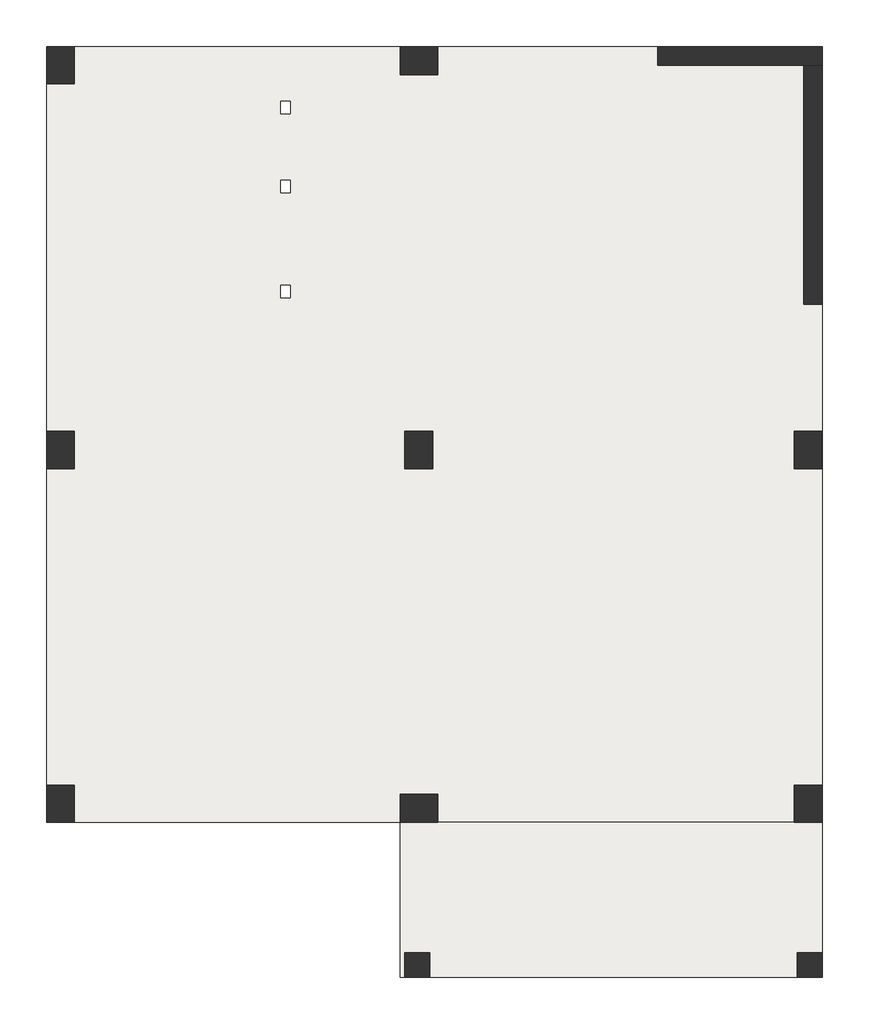
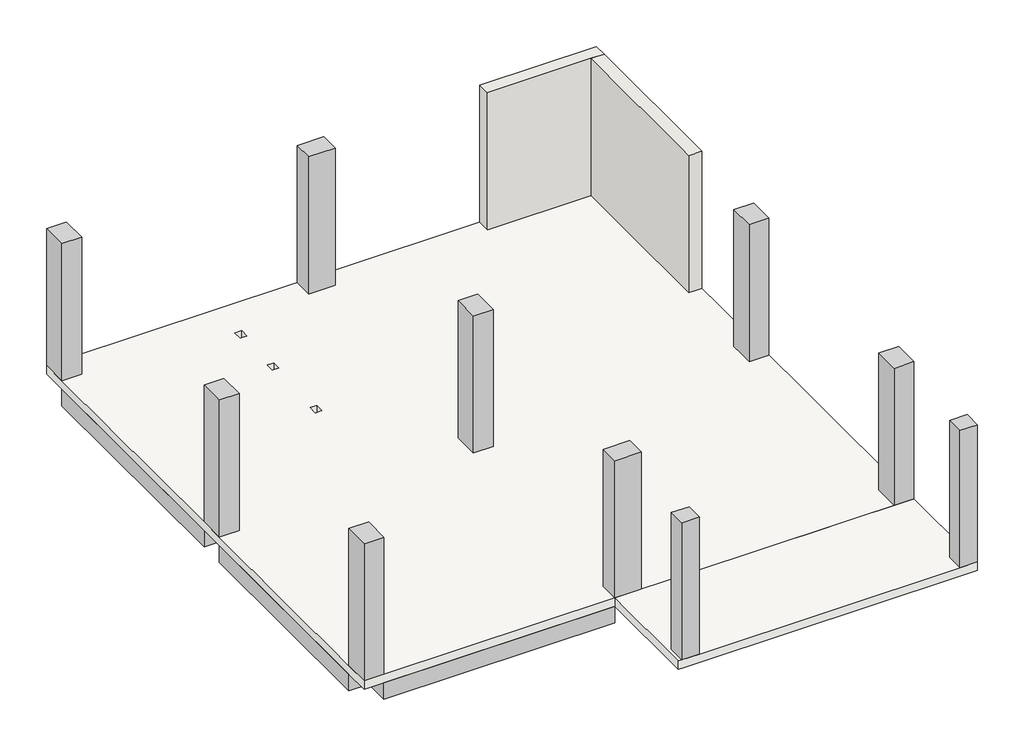
# One storey: 12 beams, 10 columns, 2 slabs, 2 walls.
"""IFC4 building model written with IfcOpenShell, lengths in millimetres."""

from ifc_helpers import new_model, si_unit, frame, origin, place, context, project, spatial, polyline, outline, extrude, faceted_brep, element, save

model = new_model("IFC4")

# Units and contexts
model_context = context("Model", 3, world=origin())
ifc_project = project(units=[si_unit("LENGTHUNIT", "METRE", prefix="MILLI")], contexts=[model_context])

# Site, building, storey
site = spatial("IfcSite", under=ifc_project)
building = spatial("IfcBuilding", under=site)
storey = spatial("IfcBuildingStorey", under=building, Name="01 Birinci Kat", Elevation=97280.0)

# Beams
placement = place(None, origin())
element("IfcBeam", 1, ObjectType="M_Concrete-Rectangular Beam : 45x60cm Kiriş", at=placement, inside=storey, context=model_context, shape_type="SweptSolid", body=[
    extrude(outline(polyline([(6225.0, 14999.2150597), (5700.0, 14999.2150597), (5700.0, 14550.0), (450.0, 14550.0), (450.0, 15000.0), (6225.0, 15000.0), (6225.0, 14999.2150597)])), frame((0.0, 0.0, 96680.0), z_axis=(0.0, 0.0, 1.0), x_axis=(1.0, 0.0, 0.0)), (0.0, 0.0, 1.0), 400.0),
])
element("IfcBeam", 2, ObjectType="M_Concrete-Rectangular Beam : 45x60cm Kiriş", at=placement, inside=storey, context=model_context, shape_type="SweptSolid", body=[
    extrude(outline(polyline([(450.0, 8750.0), (5775.0, 8750.0), (5775.0, 8300.0), (450.0, 8300.0), (450.0, 8750.0)])), frame((0.0, 0.0, 96680.0), z_axis=(0.0, 0.0, 1.0), x_axis=(1.0, 0.0, 0.0)), (0.0, 0.0, 1.0), 400.0),
])
element("IfcBeam", 3, ObjectType="M_Concrete-Rectangular Beam : 45x60cm Kiriş", at=placement, inside=storey, context=model_context, shape_type="SweptSolid", body=[
    extrude(outline(polyline([(0.0, 8800.0), (0.0, 14400.0), (450.0, 14400.0), (450.0, 8800.0), (0.0, 8800.0)])), frame((0.0, 0.0, 96680.0), z_axis=(0.0, 0.0, 1.0), x_axis=(1.0, 0.0, 0.0)), (0.0, 0.0, 1.0), 400.0),
])
element("IfcBeam", 4, ObjectType="M_Concrete-Rectangular Beam : 45x60cm Kiriş", at=placement, inside=storey, context=model_context, shape_type="SweptSolid", body=[
    extrude(outline(polyline([(0.0, 3100.0), (0.0, 8200.0), (450.0, 8200.0), (450.0, 3100.0), (0.0, 3100.0)])), frame((0.0, 0.0, 96680.0), z_axis=(0.0, 0.0, 1.0), x_axis=(1.0, 0.0, 0.0)), (0.0, 0.0, 1.0), 400.0),
])
element("IfcBeam", 5, ObjectType="M_Concrete-Rectangular Beam : 45x60cm Kiriş", at=placement, inside=storey, context=model_context, shape_type="SweptSolid", body=[
    extrude(outline(polyline([(5700.0, 2500.0), (450.0, 2500.0), (450.0, 2950.0), (5700.0, 2950.0), (5700.0, 2500.0)])), frame((0.0, 0.0, 96680.0), z_axis=(0.0, 0.0, 1.0), x_axis=(1.0, 0.0, 0.0)), (0.0, 0.0, 1.0), 400.0),
])
element("IfcBeam", 6, ObjectType="M_Concrete-Rectangular Beam : 45x60cm Kiriş", at=placement, inside=storey, context=model_context, shape_type="SweptSolid", body=[
    extrude(outline(polyline([(12050.0, 2500.0), (6300.0, 2500.0), (6300.0, 2950.0), (12050.0, 2950.0), (12050.0, 2500.0)])), frame((0.0, 0.0, 96680.0), z_axis=(0.0, 0.0, 1.0), x_axis=(1.0, 0.0, 0.0)), (0.0, 0.0, 1.0), 400.0),
])
element("IfcBeam", 7, ObjectType="M_Concrete-Rectangular Beam : 45x60cm Kiriş", at=placement, inside=storey, context=model_context, shape_type="SweptSolid", body=[
    extrude(outline(polyline([(12500.0, 8750.0), (12500.0, 3100.0), (12050.0, 3100.0), (12050.0, 8200.0), (12494.8117928, 8200.0), (12494.8117928, 8750.0), (12500.0, 8750.0)])), frame((0.0, 0.0, 96680.0), z_axis=(0.0, 0.0, 1.0), x_axis=(1.0, 0.0, 0.0)), (0.0, 0.0, 1.0), 400.0),
])
element("IfcBeam", 8, ObjectType="M_Concrete-Rectangular Beam : 45x60cm Kiriş", at=placement, inside=storey, context=model_context, shape_type="SweptSolid", body=[
    extrude(outline(polyline([(12044.8117928, 8750.0), (12044.8117928, 8300.0), (6237.7, 8300.0), (6237.7, 8750.0), (12044.8117928, 8750.0)])), frame((0.0, 0.0, 96680.0), z_axis=(0.0, 0.0, 1.0), x_axis=(1.0, 0.0, 0.0)), (0.0, 0.0, 1.0), 400.0),
])
element("IfcBeam", 9, ObjectType="M_Concrete-Rectangular Beam : 30x60cm Kiriş", at=placement, inside=storey, context=model_context, shape_type="SweptSolid", body=[
    extrude(outline(polyline([(9850.0, 15000.0), (9850.0, 14700.0), (6300.0, 14700.0), (6300.0, 15000.0), (9850.0, 15000.0)])), frame((0.0, 0.0, 96680.0), z_axis=(0.0, 0.0, 1.0), x_axis=(1.0, 0.0, 0.0)), (0.0, 0.0, 1.0), 400.0),
])
element("IfcBeam", 10, ObjectType="M_Concrete-Rectangular Beam : 30x60cm Kiriş", at=placement, inside=storey, context=model_context, shape_type="SweptSolid", body=[
    extrude(outline(polyline([(12200.0, 10850.0), (12500.0, 10850.0), (12500.0, 8800.0), (12200.0, 8800.0), (12200.0, 10850.0)])), frame((0.0, 0.0, 96680.0), z_axis=(0.0, 0.0, 1.0), x_axis=(1.0, 0.0, 0.0)), (0.0, 0.0, 1.0), 400.0),
])
element("IfcBeam", 11, ObjectType="M_Concrete-Rectangular Beam : 45x60cm Kiriş", at=placement, inside=storey, context=model_context, shape_type="SweptSolid", body=[
    extrude(outline(polyline([(5775.0, 2950.0), (5775.0, 8200.0), (6225.0, 8200.0), (6225.0, 2950.0), (5775.0, 2950.0)])), frame((0.0, 0.0, 96680.0), z_axis=(0.0, 0.0, 1.0), x_axis=(1.0, 0.0, 0.0)), (0.0, 0.0, 1.0), 400.0),
])
element("IfcBeam", 12, ObjectType="M_Concrete-Rectangular Beam : 45x60cm Kiriş", at=placement, inside=storey, context=model_context, shape_type="SweptSolid", body=[
    extrude(outline(polyline([(5775.0, 14536.5150597), (6225.0, 14536.5150597), (6225.0, 8800.0), (5775.0, 8800.0), (5775.0, 14536.5150597)])), frame((0.0, 0.0, 96680.0), z_axis=(0.0, 0.0, 1.0), x_axis=(1.0, 0.0, 0.0)), (0.0, 0.0, 1.0), 400.0),
])

# Columns
element("IfcColumn", 13, ObjectType="M_Concrete-Rectangular-Column : 45x60cm Kolon", at=placement, inside=storey, context=model_context, shape_type="SweptSolid", body=[
    extrude(outline(polyline([(0.0, 14400.0), (0.0, 15000.0), (450.0, 15000.0), (450.0, 14400.0), (0.0, 14400.0)])), frame((0.0, 0.0, 97280.0), z_axis=(0.0, 0.0, 1.0), x_axis=(1.0, 0.0, 0.0)), (0.0, 0.0, 1.0), 3300.0),
])
element("IfcColumn", 14, ObjectType="M_Concrete-Rectangular-Column : 45x60cm Kolon", at=placement, inside=storey, context=model_context, shape_type="SweptSolid", body=[
    extrude(outline(polyline([(5700.0, 14999.2150597), (6300.0, 14999.2150597), (6300.0, 14549.2150597), (5700.0, 14549.2150597), (5700.0, 14999.2150597)])), frame((0.0, 0.0, 97280.0), z_axis=(0.0, 0.0, 1.0), x_axis=(1.0, 0.0, 0.0)), (0.0, 0.0, 1.0), 3300.0),
])
element("IfcColumn", 15, ObjectType="M_Concrete-Rectangular-Column : 45x60cm Kolon", at=placement, inside=storey, context=model_context, shape_type="SweptSolid", body=[
    extrude(outline(polyline([(450.0, 8800.0), (450.0, 8200.0), (0.0, 8200.0), (0.0, 8800.0), (450.0, 8800.0)])), frame((0.0, 0.0, 97280.0), z_axis=(0.0, 0.0, 1.0), x_axis=(1.0, 0.0, 0.0)), (0.0, 0.0, 1.0), 3300.0),
])
element("IfcColumn", 16, ObjectType="M_Concrete-Rectangular-Column : 45x60cm Kolon", at=placement, inside=storey, context=model_context, shape_type="SweptSolid", body=[
    extrude(outline(polyline([(6225.0, 8800.0), (6225.0, 8200.0), (5775.0, 8200.0), (5775.0, 8800.0), (6225.0, 8800.0)])), frame((0.0, 0.0, 97280.0), z_axis=(0.0, 0.0, 1.0), x_axis=(1.0, 0.0, 0.0)), (0.0, 0.0, 1.0), 3300.0),
])
element("IfcColumn", 17, ObjectType="M_Concrete-Rectangular-Column : 45x60cm Kolon", at=placement, inside=storey, context=model_context, shape_type="SweptSolid", body=[
    extrude(outline(polyline([(12494.8117928, 8800.0), (12494.8117928, 8200.0), (12044.8117928, 8200.0), (12044.8117928, 8800.0), (12494.8117928, 8800.0)])), frame((0.0, 0.0, 97280.0), z_axis=(0.0, 0.0, 1.0), x_axis=(1.0, 0.0, 0.0)), (0.0, 0.0, 1.0), 3300.0),
])
element("IfcColumn", 18, ObjectType="M_Concrete-Rectangular-Column : 45x60cm Kolon", at=placement, inside=storey, context=model_context, shape_type="SweptSolid", body=[
    extrude(outline(polyline([(12500.0, 3100.0), (12500.0, 2500.0), (12050.0, 2500.0), (12050.0, 3100.0), (12500.0, 3100.0)])), frame((0.0, 0.0, 97280.0), z_axis=(0.0, 0.0, 1.0), x_axis=(1.0, 0.0, 0.0)), (0.0, 0.0, 1.0), 3300.0),
])
element("IfcColumn", 19, ObjectType="M_Concrete-Rectangular-Column : 45x60cm Kolon", at=placement, inside=storey, context=model_context, shape_type="SweptSolid", body=[
    extrude(outline(polyline([(450.0, 3100.0), (450.0, 2500.0), (0.0, 2500.0), (0.0, 3100.0), (450.0, 3100.0)])), frame((0.0, 0.0, 97280.0), z_axis=(0.0, 0.0, 1.0), x_axis=(1.0, 0.0, 0.0)), (0.0, 0.0, 1.0), 3300.0),
])
element("IfcColumn", 20, ObjectType="M_Concrete-Rectangular-Column : 45x60cm Kolon", at=placement, inside=storey, context=model_context, shape_type="SweptSolid", body=[
    extrude(outline(polyline([(5700.0, 2950.0), (6300.0, 2950.0), (6300.0, 2500.0), (5700.0, 2500.0), (5700.0, 2950.0)])), frame((0.0, 0.0, 97280.0), z_axis=(0.0, 0.0, 1.0), x_axis=(1.0, 0.0, 0.0)), (0.0, 0.0, 1.0), 3300.0),
])
element("IfcColumn", 21, ObjectType="M_Concrete-Rectangular-Column : 40x40cm Kolon", at=placement, inside=storey, context=model_context, shape_type="SweptSolid", body=[
    extrude(outline(polyline([(6175.0, 400.0), (6175.0, 0.0), (5775.0, 0.0), (5775.0, 400.0), (6175.0, 400.0)])), frame((0.0, 0.0, 97280.0), z_axis=(0.0, 0.0, 1.0), x_axis=(1.0, 0.0, 0.0)), (0.0, 0.0, 1.0), 3300.0),
])
element("IfcColumn", 22, ObjectType="M_Concrete-Rectangular-Column : 40x40cm Kolon", at=placement, inside=storey, context=model_context, shape_type="SweptSolid", body=[
    extrude(outline(polyline([(12500.0, 400.0), (12500.0, 0.0), (12100.0, 0.0), (12100.0, 400.0), (12500.0, 400.0)])), frame((0.0, 0.0, 97280.0), z_axis=(0.0, 0.0, 1.0), x_axis=(1.0, 0.0, 0.0)), (0.0, 0.0, 1.0), 3300.0),
])

# Slabs
element("IfcSlab", 23, ObjectType="20cm Döşeme", at=placement, inside=storey, context=model_context, shape_type="Brep", body=[
    faceted_brep([(12500.0, 15000.0, 97080.0), (12500.0, 10850.0, 97080.0), (12500.0, 8800.0, 97080.0), (12500.0, 8750.0, 97080.0), (12500.0, 3100.0, 97080.0), (12500.0, 2500.0, 97080.0), (12050.0, 2500.0, 97080.0), (6300.0, 2500.0, 97080.0), (5700.0, 2500.0, 97080.0), (450.0, 2500.0, 97080.0), (0.0, 2500.0, 97080.0), (0.0, 3100.0, 97080.0), (0.0, 8200.0, 97080.0), (0.0, 8800.0, 97080.0), (0.0, 14400.0, 97080.0), (0.0, 15000.0, 97080.0), (450.0, 15000.0, 97080.0), (6225.0, 15000.0, 97080.0), (6300.0, 15000.0, 97080.0), (9850.0, 15000.0, 97080.0), (3925.0, 14120.0, 97080.0), (3775.0, 14120.0, 97080.0), (3775.0, 13920.0, 97080.0), (3925.0, 13920.0, 97080.0), (3925.0, 12846.5789726, 97080.0), (3775.0, 12846.5789726, 97080.0), (3775.0, 12646.5789726, 97080.0), (3925.0, 12646.5789726, 97080.0), (3775.0, 10954.975, 97080.0), (3925.0, 10954.975, 97080.0), (3925.0, 11154.975, 97080.0), (3775.0, 11154.975, 97080.0), (12500.0, 15000.0, 97280.0), (450.0, 15000.0, 97280.0), (0.0, 15000.0, 97280.0), (0.0, 14400.0, 97280.0), (0.0, 8800.0, 97280.0), (0.0, 8200.0, 97280.0), (0.0, 3100.0, 97280.0), (0.0, 2500.0, 97280.0), (450.0, 2500.0, 97280.0), (5700.0, 2500.0, 97280.0), (6300.0, 2500.0, 97280.0), (12050.0, 2500.0, 97280.0), (12500.0, 2500.0, 97280.0), (12500.0, 3100.0, 97280.0), (3925.0, 14120.0, 97280.0), (3925.0, 13920.0, 97280.0), (3775.0, 13920.0, 97280.0), (3775.0, 14120.0, 97280.0), (3925.0, 12846.5789726, 97280.0), (3925.0, 12646.5789726, 97280.0), (3775.0, 12646.5789726, 97280.0), (3775.0, 12846.5789726, 97280.0), (3775.0, 10954.975, 97280.0), (3775.0, 11154.975, 97280.0), (3925.0, 11154.975, 97280.0), (3925.0, 10954.975, 97280.0)], [[[0, 1, 2, 3, 4, 5, 6, 7, 8, 9, 10, 11, 12, 13, 14, 15, 16, 17, 18, 19], [20, 21, 22, 23], [24, 25, 26, 27], [28, 29, 30, 31]], [[32, 33, 34, 35, 36, 37, 38, 39, 40, 41, 42, 43, 44, 45], [46, 47, 48, 49], [50, 51, 52, 53], [54, 55, 56, 57]], [[5, 4, 3, 2, 1, 0, 32, 45, 44]], [[10, 9, 8, 7, 6, 5, 44, 43, 42, 41, 40, 39]], [[15, 14, 13, 12, 11, 10, 39, 38, 37, 36, 35, 34]], [[0, 19, 18, 17, 16, 15, 34, 33, 32]], [[21, 20, 46, 49]], [[22, 21, 49, 48]], [[23, 22, 48, 47]], [[20, 23, 47, 46]], [[25, 24, 50, 53]], [[26, 25, 53, 52]], [[27, 26, 52, 51]], [[24, 27, 51, 50]], [[29, 28, 54, 57]], [[30, 29, 57, 56]], [[31, 30, 56, 55]], [[28, 31, 55, 54]]]),
])
element("IfcSlab", 24, ObjectType="20cm Döşeme", at=placement, inside=storey, context=model_context, shape_type="Brep", body=[
    faceted_brep([(12500.0, 2500.0, 97080.0), (12500.0, 450.0, 97080.0), (12500.0, 0.0, 97080.0), (12050.0, 0.0, 97080.0), (6225.0, 0.0, 97080.0), (5775.0, 0.0, 97080.0), (5700.0, 0.0, 97080.0), (5700.0, 2500.0, 97080.0), (12500.0, 2500.0, 97280.0), (5700.0, 2500.0, 97280.0), (5700.0, 0.0, 97280.0), (5775.0, 0.0, 97280.0), (6175.0, 0.0, 97280.0), (12100.0, 0.0, 97280.0), (12500.0, 0.0, 97280.0), (12500.0, 400.0, 97280.0)], [[[0, 1, 2, 3, 4, 5, 6, 7]], [[8, 9, 10, 11, 12, 13, 14, 15]], [[2, 1, 0, 8, 15, 14]], [[6, 5, 4, 3, 2, 14, 13, 12, 11, 10]], [[7, 6, 10, 9]], [[0, 7, 9, 8]]]),
])

# Walls
element("IfcWall", 25, ObjectType="30cm Perde Duvar", at=placement, inside=storey, context=model_context, shape_type="Brep", body=[
    faceted_brep([(9850.0, 14700.0, 97280.0), (12200.0, 14700.0, 97280.0), (12500.0, 14700.0, 97280.0), (12500.0, 14700.0, 100580.0), (12200.0, 14700.0, 100580.0), (9850.0, 14700.0, 100580.0), (9850.0, 14700.0, 100180.0), (9850.0, 15000.0, 97280.0), (9850.0, 15000.0, 100180.0), (9850.0, 15000.0, 100580.0), (12500.0, 15000.0, 100580.0), (12500.0, 15000.0, 97280.0)], [[[0, 1, 2, 3, 4, 5, 6]], [[7, 8, 9, 10, 11]], [[2, 1, 0, 7, 11]], [[0, 6, 5, 9, 8, 7]], [[3, 2, 11, 10]], [[5, 4, 3, 10, 9]]]),
])
element("IfcWall", 26, ObjectType="30cm Perde Duvar", at=placement, inside=storey, context=model_context, shape_type="Brep", body=[
    faceted_brep([(12200.0, 14700.0, 97280.0), (12200.0, 10850.0, 97280.0), (12200.0, 10850.0, 100180.0), (12200.0, 10850.0, 100580.0), (12200.0, 14700.0, 100580.0), (12500.0, 14700.0, 97280.0), (12500.0, 14700.0, 100580.0), (12500.0, 10850.0, 100580.0), (12500.0, 10850.0, 100180.0), (12500.0, 10850.0, 97280.0)], [[[0, 1, 2, 3, 4]], [[5, 6, 7, 8, 9]], [[1, 0, 5, 9]], [[3, 2, 1, 9, 8, 7]], [[0, 4, 6, 5]], [[4, 3, 7, 6]]]),
])

save(model, "model.ifc")

# Revit data of these elements
# Type "M_Concrete-Rectangular Beam : 45x60cm Kiriş"
#   Length [instance default] = 152.40 cm
#   b = 45.00 cm
#   h = 60.00 cm
#   Structural Material [instance default] = Concrete, Cast-in-Place gray
#   Assembly Code = ""
# Type "M_Concrete-Rectangular Beam : 30x60cm Kiriş"
#   Length [instance default] = 152.40 cm
#   b = 30.00 cm
#   h = 60.00 cm
#   Structural Material [instance default] = Concrete, Cast-in-Place gray
#   Assembly Code = ""
# Type "M_Concrete-Rectangular-Column : 45x60cm Kolon"
#   b = 45.00 cm
#   h = 60.00 cm
#   Structural Material [instance default] = Concrete, Cast-in-Place gray
# Type "M_Concrete-Rectangular-Column : 40x40cm Kolon"
#   b = 40.00 cm
#   h = 40.00 cm
#   Structural Material [instance default] = Concrete, Cast-in-Place gray
# Type "20cm Döşeme"
#   Function = 0
#   Layers, outside or top first: 20.00 cm "Concrete, Cast In Situ" (function 1)
# Type "30cm Perde Duvar"
#   Layers, outside or top first: 30.00 cm "Concrete, Cast In Situ" (function 1)
# Elements 1, 2, 3, 4, 5, 6, 7, 8, 11, 12 (IfcBeam, "M_Concrete-Rectangular Beam : 45x60cm Kiriş")
#   Comments = ""
#   Structural Material = Concrete, Cast-in-Place gray
#   Phase Created = New Construction
#   Materials on its faces: "Concrete, Cast-in-Place gray"
# Elements 9, 10 (IfcBeam, "M_Concrete-Rectangular Beam : 30x60cm Kiriş")
#   Comments = ""
#   Structural Material = Concrete, Cast-in-Place gray
#   Phase Created = New Construction
#   Materials on its faces: "Concrete, Cast-in-Place gray"
# Elements 13, 14, 15, 16, 17, 18, 19, 20 (IfcColumn, "M_Concrete-Rectangular-Column : 45x60cm Kolon")
#   Comments = ""
#   Structural Material = Concrete, Cast-in-Place gray
#   Phase Created = New Construction
#   Materials on its faces: "Concrete, Cast-in-Place gray"
# Elements 21, 22 (IfcColumn, "M_Concrete-Rectangular-Column : 40x40cm Kolon")
#   Comments = ""
#   Structural Material = Concrete, Cast-in-Place gray
#   Phase Created = New Construction
#   Materials on its faces: "Concrete, Cast-in-Place gray"
# Elements 23, 24 (IfcSlab, "20cm Döşeme")
#   Height Offset From Level = 0.00 cm
#   built-in parameter 1001954 = 1
#   Phase Created = New Construction
#   Materials on its faces: "Concrete, Cast In Situ"
# Elements 25, 26 (IfcWall, "30cm Perde Duvar")
#   Comments = ""
#   Top Offset = 0.00 cm
#   Base Offset = 0.00 cm
#   wall height = 330.00 cm
#   Phase Created = New Construction
#   Base Constraint = 01 Birinci Kat
#   Top Constraint = 02 Çatı Katı
#   Materials on its faces: "Concrete, Cast In Situ"
# Materials
#   "Concrete, Cast-in-Place gray": class "Concrete", colour RGB 192 192 192, transparency 0, Description = "Cast-in-place concrete", Cost = 0
#   "Concrete, Cast In Situ": class "Concrete", colour RGB 192 192 192, transparency 0, Description = "physical material", Cost = 0
